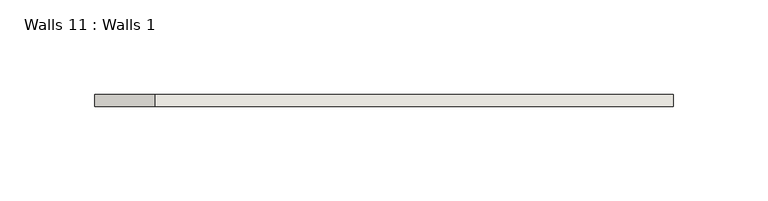
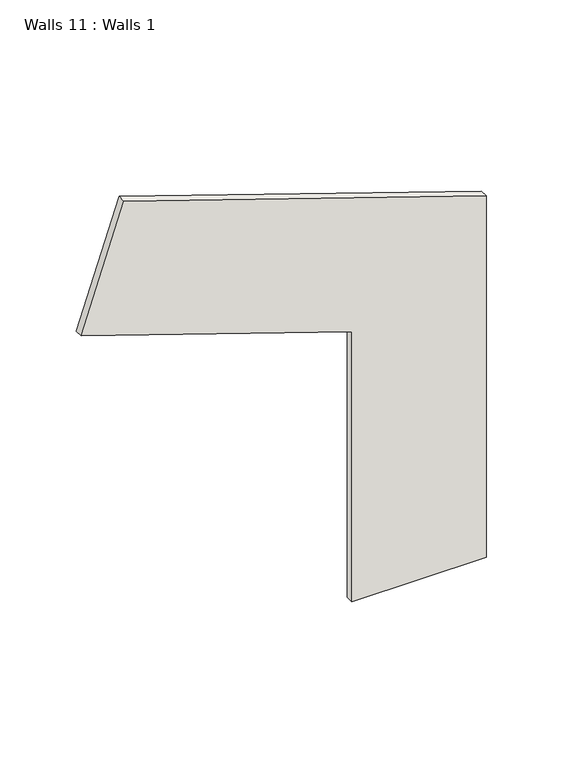
"""IFC4 building model written with IfcOpenShell, lengths in millimetres: wall geometry, Walls 11 : Walls 1."""

from ifc_helpers import new_model, si_unit, frame, origin, place, context, project, spatial, polyline, outline, extrude, source, transform, mapped, element, save


def walls_11_walls_1_f22ae6f3(model_context):
    return source(origin(), model_context, "Body", "SweptSolid", [
        extrude(outline(polyline([(5071.1413299, 23121.1370052), (5162.8996939, 22847.0612355), (5066.5557127, 22814.8060453), (4998.0134335, 23019.5370052), (4782.1134335, 23019.5370052), (4782.1134335, 23121.1370052), (5071.1413299, 23121.1370052)])), frame((0.0, -976.6384634, 0.0), z_axis=(0.0, 1.0, 0.0), x_axis=(0.0, 0.0, 1.0)), (0.0, 0.0, 1.0), 6.35),
    ])


if __name__ == "__main__":
    model = new_model("IFC4")
    model_context = context("Model", 3, world=origin())
    ifc_project = project(units=[si_unit("LENGTHUNIT", "METRE", prefix="MILLI")], contexts=[model_context])
    site = spatial("IfcSite", under=ifc_project)
    building = spatial("IfcBuilding", under=site)
    placement = place(None, origin())
    walls_11_walls_1_shape = walls_11_walls_1_f22ae6f3(model_context)
    element("IfcWall", 1, ObjectType="Walls 11 : Walls 1", at=placement, inside=building, context=model_context, shape_type="MappedRepresentation", body=[
        mapped(walls_11_walls_1_shape, transform((0.0, 0.0, 0.0), x_axis=(1.0, 0.0, 0.0), y_axis=(0.0, 1.0, 0.0), z_axis=(0.0, 0.0, 1.0))),
    ])
    save(model, "model.ifc")

# Revit data of these elements
# Element 1 (IfcWall, "Walls 11 : Walls 1")
#   Materials on its faces: "1/4\" STEEL GUSSET PLATE - (RAW STEEL)"
# Materials
#   "1/4\" STEEL GUSSET PLATE - (RAW STEEL)": class "Metal", colour RGB 189 187 185, transparency 0, Description = "Structural steel 50ksi", Cost = 0
